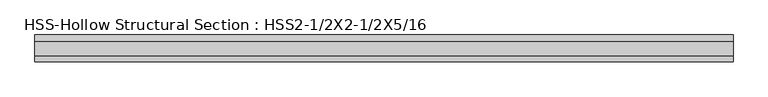
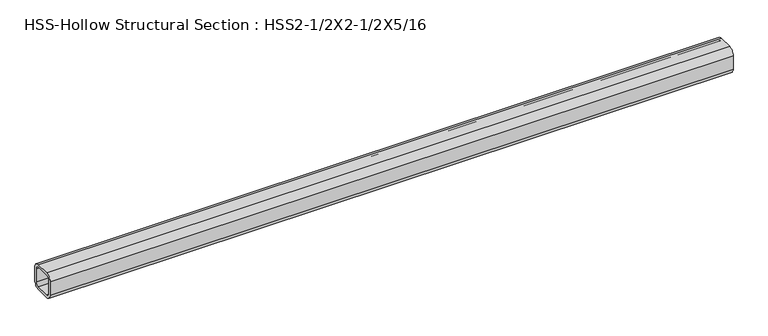
"""IFC4 building model written with IfcOpenShell, lengths in millimetres: beam geometry, HSS-Hollow Structural Section : HSS2-1/2X2-1/2X5/16."""

from ifc_helpers import new_model, si_unit, point, frame, frame_2d, origin, place, context, project, spatial, polyline, circle_curve, trimmed, segment, composite_curve, outline, extrude, source, transform, mapped, element, save


def hss_hollow_structural_section_hss2_1_2x2_1_2x5_16_d67e9168(model_context):
    return source(origin(), model_context, "Body", "SweptSolid", [
        extrude(outline(composite_curve([segment(polyline([(31.75, 16.9672), (31.75, -16.9672)]), True, "CONTINUOUS"), segment(trimmed(circle_curve(frame_2d((16.9672, -16.9672)), 14.7828), [point((31.75, -16.9672))], [point((16.9672, -31.75))], False, "CARTESIAN"), True, "CONTINUOUS"), segment(polyline([(16.9672, -31.75), (-16.9672, -31.75)]), True, "CONTINUOUS"), segment(trimmed(circle_curve(frame_2d((-16.9672, -16.9672)), 14.7828), [point((-16.9672, -31.75))], [point((-31.75, -16.9672))], False, "CARTESIAN"), True, "CONTINUOUS"), segment(polyline([(-31.75, -16.9672), (-31.75, 16.9672)]), True, "CONTINUOUS"), segment(trimmed(circle_curve(frame_2d((-16.9672, 16.9672)), 14.7828), [point((-31.75, 16.9672))], [point((-16.9672, 31.75))], False, "CARTESIAN"), True, "CONTINUOUS"), segment(polyline([(-16.9672, 31.75), (16.9672, 31.75)]), True, "CONTINUOUS"), segment(trimmed(circle_curve(frame_2d((16.9672, 16.9672)), 14.7828), [point((16.9672, 31.75))], [point((31.75, 16.9672))], False, "CARTESIAN"), True, "CONTINUOUS")], self_intersect=False), holes=[composite_curve([segment(trimmed(circle_curve(frame_2d((-16.9672, 16.9672)), 7.3914), [point((-16.9672, 24.3586))], [point((-24.3586, 16.9672))], True, "CARTESIAN"), True, "CONTINUOUS"), segment(polyline([(-24.3586, 16.9672), (-24.3586, -16.9672)]), True, "CONTINUOUS"), segment(trimmed(circle_curve(frame_2d((-16.9672, -16.9672)), 7.3914), [point((-24.3586, -16.9672))], [point((-16.9672, -24.3586))], True, "CARTESIAN"), True, "CONTINUOUS"), segment(polyline([(-16.9672, -24.3586), (16.9672, -24.3586)]), True, "CONTINUOUS"), segment(trimmed(circle_curve(frame_2d((16.9672, -16.9672)), 7.3914), [point((16.9672, -24.3586))], [point((24.3586, -16.9672))], True, "CARTESIAN"), True, "CONTINUOUS"), segment(polyline([(24.3586, -16.9672), (24.3586, 16.9672)]), True, "CONTINUOUS"), segment(trimmed(circle_curve(frame_2d((16.9672, 16.9672)), 7.3914), [point((24.3586, 16.9672))], [point((16.9672, 24.3586))], True, "CARTESIAN"), True, "CONTINUOUS"), segment(polyline([(16.9672, 24.3586), (-16.9672, 24.3586)]), True, "CONTINUOUS")], self_intersect=False)]), frame((-825.5, 0.0, 0.0), z_axis=(1.0, 0.0, 0.0), x_axis=(0.0, 1.0, 0.0)), (0.0, 0.0, 1.0), 1651.0),
    ])


if __name__ == "__main__":
    model = new_model("IFC4")
    model_context = context("Model", 3, world=origin())
    ifc_project = project(units=[si_unit("LENGTHUNIT", "METRE", prefix="MILLI")], contexts=[model_context])
    site = spatial("IfcSite", under=ifc_project)
    building = spatial("IfcBuilding", under=site)
    placement = place(None, origin())
    hss_hollow_structural_section_hss2_1_2x2_1_2x5_16_shape = hss_hollow_structural_section_hss2_1_2x2_1_2x5_16_d67e9168(model_context)
    element("IfcBeam", 1, ObjectType="HSS-Hollow Structural Section : HSS2-1/2X2-1/2X5/16", at=placement, inside=building, context=model_context, shape_type="MappedRepresentation", body=[
        mapped(hss_hollow_structural_section_hss2_1_2x2_1_2x5_16_shape, transform((0.0, 0.0, 0.0), x_axis=(1.0, 0.0, 0.0), y_axis=(0.0, 1.0, 0.0), z_axis=(0.0, 0.0, 1.0))),
    ])
    save(model, "model.ifc")

# Revit data of these elements
# Type "HSS-Hollow Structural Section : HSS2-1/2X2-1/2X5/16"
#   Assembly Code = "B10"
#   Shape = "Square"
#   W = 8.4
#   Ht = 0' - 2 1/2"
#   Length [instance default] = 5' - 0"
#   b = 0' - 2 1/2"
#   kr = 0' - 0.582"
#   t = 0' - 0.291"
#   A = 0.0163194 SF
#   Structural Material [instance default] = Steel ASTM A500, Grade B, Rectangular and Square
# Element 1 (IfcBeam, "HSS-Hollow Structural Section : HSS2-1/2X2-1/2X5/16")
#   Materials on its faces: "Steel ASTM A500, Grade B, Rectangular and Square"
# Materials
#   "Steel ASTM A500, Grade B, Rectangular and Square": class "Metal", colour RGB 199 199 199, transparency 0, Description = "Carbon steel", Cost = 0
